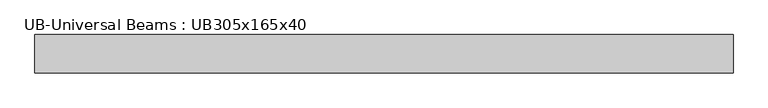
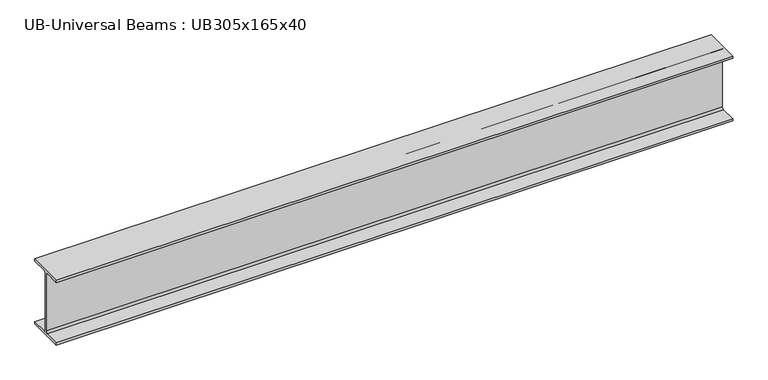
"""IFC4 building model written with IfcOpenShell, lengths in millimetres: beam geometry, UB-Universal Beams : UB305x165x40."""

import ifcopenshell
import ifcopenshell.guid

model = None  # the IFC model being written
_history = None  # IfcOwnerHistory: only IFC2X3 demands one
_inside = {}  # id of a spatial element -> (the spatial element, [elements in it])
_under = {}  # id of a project, library or spatial element -> (it, [spatial elements below it])
_declared = {}  # id of a project -> (the project, [libraries it declares])
_typed = {}  # id of a type object -> (the type object, [elements of that type])
_made_of = {}  # id of a material, layer set ... -> (it, [elements and type objects made of it])


def new_model(schema):
    """Start an empty IFC model of exactly this schema.

    Asked for "IFC4X3", IfcOpenShell would pick the latest addendum, in which some entities
    have other attributes; the version numbers below select the first issue.
    IFC2X3 requires an IfcOwnerHistory on every rooted entity: one is made here for all.
    """
    global model, _history
    if schema == "IFC4X3":
        model = ifcopenshell.file(schema_version=(4, 3, 0, 0))
    else:
        model = ifcopenshell.file(schema=schema)
    _inside.clear()
    _under.clear()
    _declared.clear()
    _typed.clear()
    _made_of.clear()
    _history = None
    if model.schema == "IFC2X3":
        org = make("IfcOrganization", Name="unknown")
        user = make(
            "IfcPersonAndOrganization",
            ThePerson=make("IfcPerson", FamilyName="unknown"),
            TheOrganization=org,
        )
        app = make(
            "IfcApplication",
            ApplicationDeveloper=org,
            Version="unknown",
            ApplicationFullName="unknown",
            ApplicationIdentifier="unknown",
        )
        _history = make(
            "IfcOwnerHistory",
            OwningUser=user,
            OwningApplication=app,
            ChangeAction="ADDED",
            CreationDate=0,
        )
    return model


def make(cls, **values):
    """One entity of the class cls with the attributes given. An attribute that is None is left unset."""
    return model.create_entity(
        cls, **{name: value for name, value in values.items() if value is not None}
    )


def rooted(cls, **values):
    """An entity with a GlobalId (a new one), such as an element, a storey or a relation."""
    return make(cls, GlobalId=ifcopenshell.guid.new(), OwnerHistory=_history, **values)


def si_unit(unit_type, name, prefix=None):
    """IfcSIUnit, for example si_unit("LENGTHUNIT", "METRE", prefix="MILLI")."""
    return make("IfcSIUnit", UnitType=unit_type, Prefix=prefix, Name=name)


def assignment(units):
    """IfcUnitAssignment: the units of a project."""
    return None if units is None else make("IfcUnitAssignment", Units=units)


def point(xyz):
    """IfcCartesianPoint."""
    return None if xyz is None else make("IfcCartesianPoint", Coordinates=xyz)


def direction(xyz):
    """IfcDirection."""
    return None if xyz is None else make("IfcDirection", DirectionRatios=xyz)


def frame(location, z_axis=None, x_axis=None):
    """IfcAxis2Placement3D, a coordinate frame: its origin and axes. An axis left out is left unset."""
    return make(
        "IfcAxis2Placement3D",
        Location=point(location),
        Axis=direction(z_axis),
        RefDirection=direction(x_axis),
    )


def frame_2d(location, x_axis=None):
    """IfcAxis2Placement2D, a coordinate frame in the plane: its origin and x axis."""
    return make(
        "IfcAxis2Placement2D", Location=point(location), RefDirection=direction(x_axis)
    )


def origin():
    """The frame at (0, 0, 0) with its axes left unset."""
    return frame((0.0, 0.0, 0.0))


def place(relative_to, where):
    """IfcLocalPlacement: puts the frame where relative to a parent placement (None: the world)."""
    return make(
        "IfcLocalPlacement", PlacementRelTo=relative_to, RelativePlacement=where
    )


def context(
    kind, dimensions, precision=None, world=None, true_north=None, identifier=None
):
    """IfcGeometricRepresentationContext, for example the 3D "Model" context."""
    return make(
        "IfcGeometricRepresentationContext",
        ContextIdentifier=identifier,
        ContextType=kind,
        CoordinateSpaceDimension=dimensions,
        Precision=precision,
        WorldCoordinateSystem=world,
        TrueNorth=true_north,
    )


def project(units=None, contexts=None):
    """IfcProject with its units and contexts."""
    return rooted(
        "IfcProject",
        Name="project",
        RepresentationContexts=contexts,
        UnitsInContext=assignment(units),
    )


def spatial(cls, under=None, at=None, **own):
    """A site, building, storey or space (cls), placed at a placement, below another one or the project."""
    s = rooted(cls, ObjectPlacement=at, **own)
    if under is not None:
        _under.setdefault(under.id(), (under, []))[1].append(s)
    return s


def polyline(points):
    """IfcPolyline through the points."""
    return make("IfcPolyline", Points=[point(p) for p in points])


def circle_curve(where, radius):
    """IfcCircle in the frame where."""
    return make("IfcCircle", Position=where, Radius=radius)


def trimmed(basis, trim1, trim2, sense, master):
    """IfcTrimmedCurve: the piece of a basis curve between two trims."""
    return make(
        "IfcTrimmedCurve",
        BasisCurve=basis,
        Trim1=trim1,
        Trim2=trim2,
        SenseAgreement=sense,
        MasterRepresentation=master,
    )


def segment(curve, same_sense, transition):
    """IfcCompositeCurveSegment."""
    return make(
        "IfcCompositeCurveSegment",
        Transition=transition,
        SameSense=same_sense,
        ParentCurve=curve,
    )


def composite_curve(segments, self_intersect=None):
    """IfcCompositeCurve: segments joined end to end."""
    return make("IfcCompositeCurve", Segments=segments, SelfIntersect=self_intersect)


def outline(outer, holes=None, kind="AREA"):
    """IfcArbitraryClosedProfileDef: a profile drawn as a closed curve; with holes, ...WithVoids."""
    if holes is None:
        return make("IfcArbitraryClosedProfileDef", ProfileType=kind, OuterCurve=outer)
    return make(
        "IfcArbitraryProfileDefWithVoids",
        ProfileType=kind,
        OuterCurve=outer,
        InnerCurves=holes,
    )


def extrude(swept, where, along, depth):
    """IfcExtrudedAreaSolid: the profile swept, set in the frame where, extruded along a direction by depth."""
    return make(
        "IfcExtrudedAreaSolid",
        SweptArea=swept,
        Position=where,
        ExtrudedDirection=direction(along),
        Depth=depth,
    )


def shape(context_of_items, identifier, shape_type, items):
    """IfcShapeRepresentation: the items that make up one representation, for example the "Body"."""
    return make(
        "IfcShapeRepresentation",
        ContextOfItems=context_of_items,
        RepresentationIdentifier=identifier,
        RepresentationType=shape_type,
        Items=items,
    )


def source(mapping_origin, context_of_items, identifier, shape_type, items):
    """IfcRepresentationMap: a shape defined once, which mapped items show again and again."""
    return make(
        "IfcRepresentationMap",
        MappingOrigin=mapping_origin,
        MappedRepresentation=shape(context_of_items, identifier, shape_type, items),
    )


def transform(
    local_origin,
    x_axis=None,
    y_axis=None,
    z_axis=None,
    scale=None,
    scale2=None,
    scale3=None,
    uniform=True,
):
    """IfcCartesianTransformationOperator3D, or its non-uniform kind. x_axis, y_axis, z_axis: its Axis1, 2, 3."""
    if uniform:
        return make(
            "IfcCartesianTransformationOperator3D",
            Axis1=direction(x_axis),
            Axis2=direction(y_axis),
            LocalOrigin=point(local_origin),
            Scale=scale,
            Axis3=direction(z_axis),
        )
    return make(
        "IfcCartesianTransformationOperator3DnonUniform",
        Axis1=direction(x_axis),
        Axis2=direction(y_axis),
        LocalOrigin=point(local_origin),
        Scale=scale,
        Axis3=direction(z_axis),
        Scale2=scale2,
        Scale3=scale3,
    )


def mapped(mapping_source, mapping_target):
    """IfcMappedItem: shows the shape of a source again, moved by a transform."""
    return make(
        "IfcMappedItem", MappingSource=mapping_source, MappingTarget=mapping_target
    )


def made_of(thing, what):
    """Note that an element or type object is made of a material, layer set ...; save() writes the relation."""
    if what is not None:
        _made_of.setdefault(what.id(), (what, []))[1].append(thing)
    return thing


def element(
    cls,
    number,
    at=None,
    inside=None,
    cuts=None,
    type_object=None,
    material=None,
    context=None,
    identifier="Body",
    shape_type=None,
    held_by="IfcProductDefinitionShape",
    body=None,
    shapes=None,
    **own,
):
    """One element of the class cls, such as IfcWall. Its Tag is "e" and its number.

    at: its placement. inside: the storey or other place that contains it. cuts: it is an
    opening in that element (IfcRelVoidsElement). A single representation is given by context,
    identifier, shape_type and body (its items); several are given by shapes. held_by: the class
    of the entity that holds the representations. save() writes the other relations.
    """
    e = rooted(cls, Tag="e%d" % number, ObjectPlacement=at, **own)
    if body is not None:
        shapes = [shape(context, identifier, shape_type, body)]
    if shapes is not None:
        e.Representation = make(held_by, Representations=shapes)
    if inside is not None:
        _inside.setdefault(inside.id(), (inside, []))[1].append(e)
    if cuts is not None:
        rooted(
            "IfcRelVoidsElement", RelatingBuildingElement=cuts, RelatedOpeningElement=e
        )
    if type_object is not None:
        _typed.setdefault(type_object.id(), (type_object, []))[1].append(e)
    return made_of(e, material)


def aggregate(whole, parts):
    """IfcRelAggregates: a whole, such as a stair, and the parts it consists of."""
    return rooted("IfcRelAggregates", RelatingObject=whole, RelatedObjects=parts)


def save(model, path):
    """Write the relations noted so far, then the file.

    IfcRelAggregates (storeys below a building ...), IfcRelContainedInSpatialStructure (elements
    in a storey), IfcRelDefinesByType, IfcRelAssociatesMaterial and IfcRelDeclares: one each for
    every whole, place, type object, material and project.
    """
    for whole, parts in _under.values():
        aggregate(whole, parts)
    for where, things in _inside.values():
        rooted(
            "IfcRelContainedInSpatialStructure",
            RelatedElements=things,
            RelatingStructure=where,
        )
    for kind, things in _typed.values():
        rooted("IfcRelDefinesByType", RelatedObjects=things, RelatingType=kind)
    for what, things in _made_of.values():
        rooted("IfcRelAssociatesMaterial", RelatedObjects=things, RelatingMaterial=what)
    for by, libraries in _declared.values():
        rooted("IfcRelDeclares", RelatingContext=by, RelatedDefinitions=libraries)
    model.write(path)


def ub_universal_beams_ub305x165x40_8b2c45c1(model_context):
    return source(origin(), model_context, "Body", "SweptSolid", [
        extrude(outline(composite_curve([segment(polyline([(82.5, -141.5), (82.5, -151.7), (-82.5, -151.7), (-82.5, -141.5), (-11.9, -141.5)]), True, "CONTINUOUS"), segment(trimmed(circle_curve(frame_2d((-11.9, -132.6)), 8.9), [point((-11.9, -141.5))], [point((-3.0, -132.6))], True, "CARTESIAN"), True, "CONTINUOUS"), segment(polyline([(-3.0, -132.6), (-3.0, 132.6)]), True, "CONTINUOUS"), segment(trimmed(circle_curve(frame_2d((-11.9, 132.6)), 8.9), [point((-3.0, 132.6))], [point((-11.9, 141.5))], True, "CARTESIAN"), True, "CONTINUOUS"), segment(polyline([(-11.9, 141.5), (-82.5, 141.5), (-82.5, 151.7), (82.5, 151.7), (82.5, 141.5), (11.9, 141.5)]), True, "CONTINUOUS"), segment(trimmed(circle_curve(frame_2d((11.9, 132.6)), 8.9), [point((11.9, 141.5))], [point((3.0, 132.6))], True, "CARTESIAN"), True, "CONTINUOUS"), segment(polyline([(3.0, 132.6), (3.0, -132.6)]), True, "CONTINUOUS"), segment(trimmed(circle_curve(frame_2d((11.9, -132.6)), 8.9), [point((3.0, -132.6))], [point((11.9, -141.5))], True, "CARTESIAN"), True, "CONTINUOUS"), segment(polyline([(11.9, -141.5), (82.5, -141.5)]), True, "CONTINUOUS")], self_intersect=False)), frame((-1500.0, 0.0, 0.0), z_axis=(1.0, 0.0, 0.0), x_axis=(0.0, 1.0, 0.0)), (0.0, 0.0, 1.0), 3000.0),
    ])


if __name__ == "__main__":
    model = new_model("IFC4")
    model_context = context("Model", 3, world=origin())
    ifc_project = project(units=[si_unit("LENGTHUNIT", "METRE", prefix="MILLI")], contexts=[model_context])
    site = spatial("IfcSite", under=ifc_project)
    building = spatial("IfcBuilding", under=site)
    placement = place(None, origin())
    ub_universal_beams_ub305x165x40_shape = ub_universal_beams_ub305x165x40_8b2c45c1(model_context)
    element("IfcBeam", 1, ObjectType="UB-Universal Beams : UB305x165x40", at=placement, inside=building, context=model_context, shape_type="MappedRepresentation", body=[
        mapped(ub_universal_beams_ub305x165x40_shape, transform((0.0, 0.0, 0.0), x_axis=(1.0, 0.0, 0.0), y_axis=(0.0, 1.0, 0.0), z_axis=(0.0, 0.0, 1.0))),
    ])
    save(model, "model.ifc")

# Revit data of these elements
# Type "UB-Universal Beams : UB305x165x40"
#   Section Name Key = "UB305X165X40"
#   Width = 16.5 cm
#   Web Thickness = 0.6 cm
#   Web Fillet = 0.89 cm
#   Warping Constant = 164000.0 cm⁶
#   Torsional Moment of Inertia = 14.70 cm⁴
#   Section Area = 51.3 cm²
#   Plastic Modulus weak axis = 142.0 cm³
#   Plastic Modulus strong axis = 623.0 cm³
#   Nominal Weight = 40.2999 kgf/m
#   Moment of Inertia weak axis = 764.00 cm⁴
#   Moment of Inertia strong axis = 8503.00 cm⁴
#   Height = 30.34 cm
#   Flange Thickness = 1.02 cm
#   Elastic Modulus weak axis = 92.6 cm³
#   Elastic Modulus strong axis = 560.0 cm³
#   Centroid Vertical = 15.17 cm
#   Centroid Horizontal = 8.25 cm
#   Bolt Spacing = 9.0 cm
#   Length [instance default] = 1500 mm
#   Structural Material [instance default] = Metal - Steel 43-275
#   Type Comments = ""
#   Assembly Code = ""
# Element 1 (IfcBeam, "UB-Universal Beams : UB305x165x40")
#   Materials on its faces: "Metal - Steel 43-275"
# Materials
#   "Metal - Steel 43-275": class "Metal", colour RGB 247 247 247, transparency 0, Cost = 0
